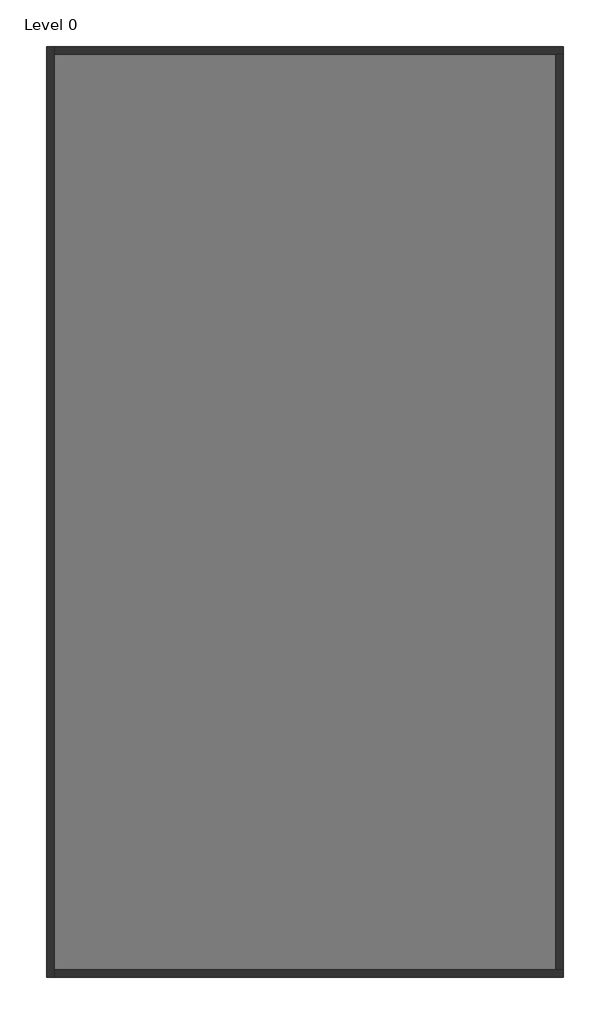
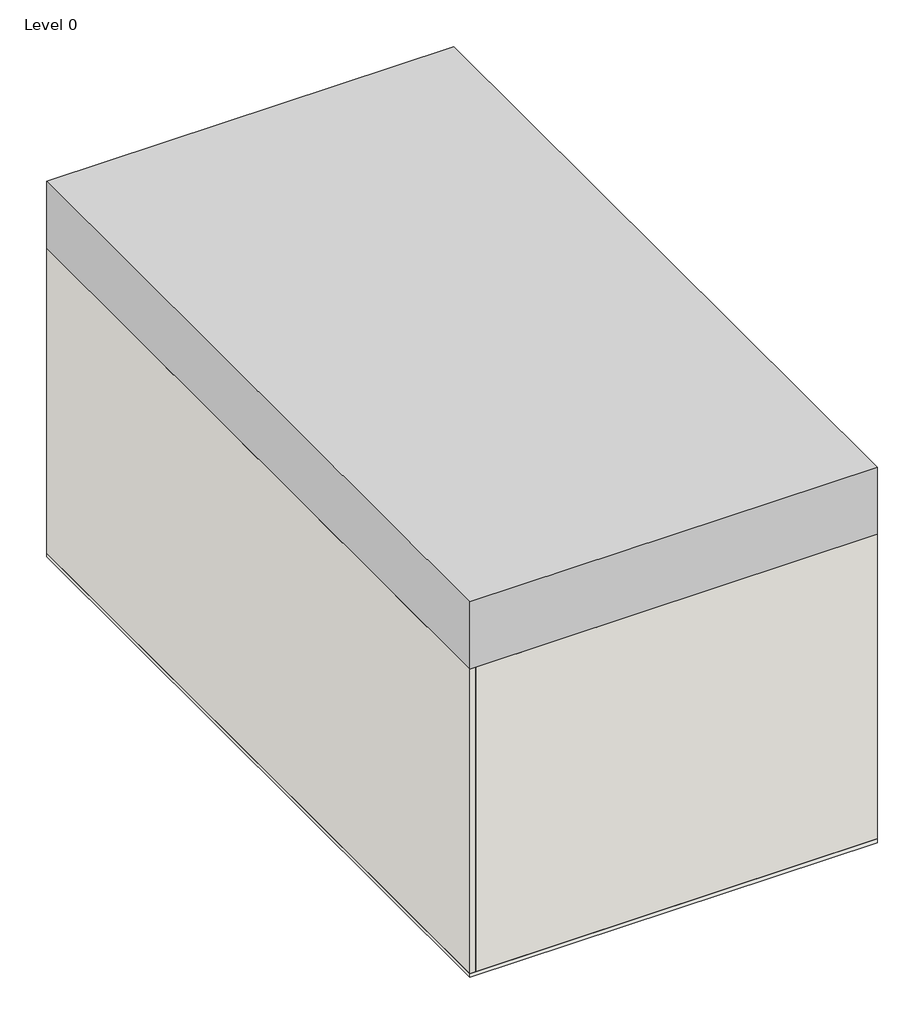
# One storey: 4 walls, 1 proxy, 1 slab.
"""IFC4 building model written with IfcOpenShell, lengths in millimetres."""

from ifc_helpers import new_model, si_unit, frame, origin, origin_with_axes, place, context, project, spatial, polyline, outline, extrude, faceted_brep, element, save

model = new_model("IFC4")

# Units and contexts
model_context = context("Model", 3, world=origin())
ifc_project = project(units=[si_unit("LENGTHUNIT", "METRE", prefix="MILLI")], contexts=[model_context])

# Site, building, storey
site = spatial("IfcSite", under=ifc_project)
building = spatial("IfcBuilding", under=site)
storey = spatial("IfcBuildingStorey", under=building, Name="Level 0", Elevation=100.0)

# Proxy
placement = place(None, origin())
element("IfcBuildingElementProxy", 1, Name="LowUrbanDensityBuilding : LowUrbanDensityBuilding", ObjectType="LowUrbanDensityBuilding : LowUrbanDensityBuilding", at=placement, inside=storey, context=model_context, shape_type="SweptSolid", body=[
    extrude(outline(polyline([(7325.2659446, 3676.2074539), (7325.2659446, -14323.7925461), (-2674.7340554, -14323.7925461), (-2674.7340554, 3676.2074539), (7325.2659446, 3676.2074539)])), origin_with_axes(), (0.0, 0.0, 1.0), 9749.8),
])

# Slab
element("IfcSlab", 2, ObjectType="Floor-Concrete_100Con", at=placement, inside=storey, context=model_context, shape_type="SweptSolid", body=[
    extrude(outline(polyline([(7325.2659446, 3676.2074539), (7325.2659446, -14323.7925461), (-2674.7340554, -14323.7925461), (-2674.7340554, 3676.2074539), (7325.2659446, 3676.2074539)])), origin_with_axes(), (0.0, 0.0, 1.0), 100.0),
])

# Walls
element("IfcWall", 3, ObjectType="Wall-Ext_25Rdr-100Blk-19P", at=placement, inside=storey, context=model_context, shape_type="Brep", body=[
    faceted_brep([(-2674.7340554, 3676.2074539, 100.0), (-2674.7340554, -14323.7925461, 100.0), (-2674.7340554, -14323.7925461, 8000.0), (-2674.7340554, 3676.2074539, 8000.0), (-2530.4340554, 3676.2074539, 100.0), (-2530.4340554, 3676.2074539, 8000.0), (-2530.4340554, 3531.9074539, 8000.0), (-2530.4340554, -14179.4925461, 8000.0), (-2530.4340554, -14323.7925461, 8000.0), (-2530.4340554, -14323.7925461, 100.0), (-2530.4340554, -14179.4925461, 100.0), (-2530.4340554, 3531.9074539, 100.0)], [[[0, 1, 2, 3]], [[4, 5, 6, 7, 8, 9, 10, 11]], [[1, 0, 4, 11, 10, 9]], [[3, 2, 8, 7, 6, 5]], [[2, 1, 9, 8]], [[0, 3, 5, 4]]]),
])
element("IfcWall", 4, ObjectType="Wall-Ext_25Rdr-100Blk-19P", at=placement, inside=storey, context=model_context, shape_type="Brep", body=[
    faceted_brep([(-2530.4340554, -14323.7925461, 100.0), (7325.2659446, -14323.7925461, 100.0), (7325.2659446, -14323.7925461, 8000.0), (-2530.4340554, -14323.7925461, 8000.0), (-2530.4340554, -14179.4925461, 100.0), (-2530.4340554, -14179.4925461, 8000.0), (7180.9659446, -14179.4925461, 8000.0), (7325.2659446, -14179.4925461, 8000.0), (7325.2659446, -14179.4925461, 100.0), (7180.9659446, -14179.4925461, 100.0)], [[[0, 1, 2, 3]], [[4, 5, 6, 7, 8, 9]], [[1, 0, 4, 9, 8]], [[3, 2, 7, 6, 5]], [[0, 3, 5, 4]], [[2, 1, 8, 7]]]),
])
element("IfcWall", 5, ObjectType="Wall-Ext_25Rdr-100Blk-19P", at=placement, inside=storey, context=model_context, shape_type="Brep", body=[
    faceted_brep([(7325.2659446, 3676.2074539, 100.0), (-2530.4340554, 3676.2074539, 100.0), (-2530.4340554, 3676.2074539, 8000.0), (7325.2659446, 3676.2074539, 8000.0), (7325.2659446, 3531.9074539, 100.0), (7325.2659446, 3531.9074539, 8000.0), (7180.9659446, 3531.9074539, 8000.0), (-2530.4340554, 3531.9074539, 8000.0), (-2530.4340554, 3531.9074539, 100.0), (7180.9659446, 3531.9074539, 100.0)], [[[0, 1, 2, 3]], [[4, 5, 6, 7, 8, 9]], [[1, 0, 4, 9, 8]], [[3, 2, 7, 6, 5]], [[2, 1, 8, 7]], [[0, 3, 5, 4]]]),
])
element("IfcWall", 6, ObjectType="Wall-Ext_25Rdr-100Blk-19P", at=placement, inside=storey, context=model_context, shape_type="SweptSolid", body=[
    extrude(outline(polyline([(7325.2659446, 3531.9074539), (7325.2659446, -14179.4925461), (7180.9659446, -14179.4925461), (7180.9659446, 3531.9074539), (7325.2659446, 3531.9074539)])), frame((0.0, 0.0, 100.0), z_axis=(0.0, 0.0, 1.0), x_axis=(1.0, 0.0, 0.0)), (0.0, 0.0, 1.0), 7900.0),
])

save(model, "model.ifc")

# Revit data of these elements
# Project information
#   Project Issue Date = "Issue Date"
#   Project Status = "Project Status"
#   Client Name = "Owner"
#   Project Address = "Enter address here"
#   Project Name = "Project Name"
#   Project Number = "Project Number"
# Type "Floor-Concrete_100Con"
#   Keynote = "E60/130"
#   Function = 0
#   Layers, outside or top first: 100 mm "Concrete" (function 1)
# Type "Wall-Ext_25Rdr-100Blk-19P"
#   Keynote = "F10"
#   Layers, outside or top first: 25.3 mm "Render, Beige, Smooth" (function 5); 100 mm "Concrete Masonry Units _Low Density" (function 1); 19 mm "Plaster" (function 5)
# Element 1 (IfcBuildingElementProxy, "LowUrbanDensityBuilding : LowUrbanDensityBuilding")
#   Phase Created = New Construction
#   Materials on its faces: "Default Form"
# Element 2 (IfcSlab, "Floor-Concrete_100Con")
#   Height Offset From Level = 0 mm
#   Phase Created = New Construction
#   Materials on its faces: "Concrete"
# Element 3 (IfcWall, "Wall-Ext_25Rdr-100Blk-19P")
#   Top Offset = 0 mm
#   Base Offset = 0 mm
#   wall height = 7900 mm
#   Phase Created = New Construction
#   Base Constraint = Level 0
#   Top Constraint = Level 2
#   Materials on its faces: "Render, Beige, Smooth", "Default Wall", "Plaster"
# Elements 4, 5, 6 (IfcWall, "Wall-Ext_25Rdr-100Blk-19P")
#   Top Offset = 0 mm
#   Base Offset = 0 mm
#   wall height = 7900 mm
#   Phase Created = New Construction
#   Base Constraint = Level 0
#   Top Constraint = Level 2
#   Materials on its faces: "Default Wall", "Render, Beige, Smooth", "Plaster"
# Materials
#   "Concrete": class "Concrete", colour RGB 120 120 120, transparency 0, Description = "Portland Cement Concrete", Cost = 0
#   "Render, Beige, Smooth": class "Generic", colour RGB 213 198 180, transparency 0, Description = "physical material", Cost = 0
#   "Concrete Masonry Units _Low Density": class "Masonry", colour RGB 181 181 181, transparency 0, Description = "Concrete masonry units", Cost = 0
#   "Plaster": class "Generic", colour RGB 249 249 249, transparency 0, Description = "Plaster", Cost = 0
#   "Default Form": class "Generic", colour RGB 185 189 196, transparency 0.5, Cost = 0
#   "Default Wall": class "Miscellaneous", colour RGB 128 128 128, transparency 0, Comments = "Rendering appearance not upgraded Rendering appearance not upgraded ", Cost = 0
